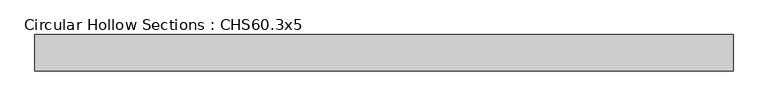
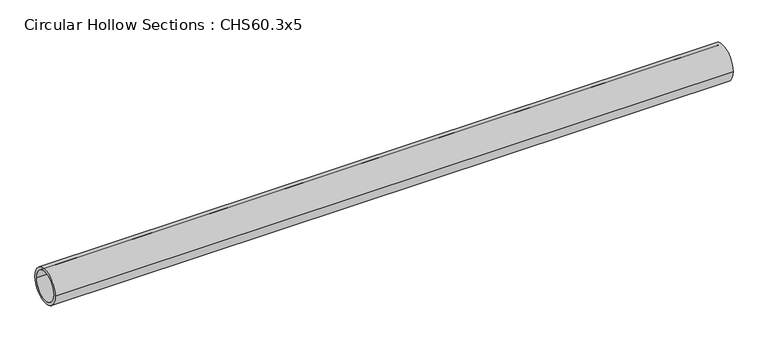
"""IFC4 building model written with IfcOpenShell, lengths in millimetres: beam geometry, Circular Hollow Sections : CHS60.3x5."""

from ifc_helpers import new_model, si_unit, point, frame, origin, origin_2d, place, context, project, spatial, circle_curve, trimmed, segment, composite_curve, outline, extrude, source, transform, mapped, element, save


def circular_hollow_sections_chs60_3x5_7809bf4e(model_context):
    return source(origin(), model_context, "Body", "SweptSolid", [
        extrude(outline(composite_curve([segment(trimmed(circle_curve(origin_2d(), 30.15), [point((-30.15, 0.0))], [point((30.15, 0.0))], False, "CARTESIAN"), True, "CONTINUOUS"), segment(trimmed(circle_curve(origin_2d(), 30.15), [point((30.15, 0.0))], [point((-30.15, 0.0))], False, "CARTESIAN"), True, "CONTINUOUS")], self_intersect=False), holes=[composite_curve([segment(trimmed(circle_curve(origin_2d(), 25.15), [point((25.15, 0.0))], [point((-25.15, 0.0))], True, "CARTESIAN"), True, "CONTINUOUS"), segment(trimmed(circle_curve(origin_2d(), 25.15), [point((-25.15, 0.0))], [point((25.15, 0.0))], True, "CARTESIAN"), True, "CONTINUOUS")], self_intersect=False)]), frame((-600.0, 0.0, 0.0), z_axis=(1.0, 0.0, 0.0), x_axis=(0.0, 1.0, 0.0)), (0.0, 0.0, 1.0), 1157.0),
    ])


if __name__ == "__main__":
    model = new_model("IFC4")
    model_context = context("Model", 3, world=origin())
    ifc_project = project(units=[si_unit("LENGTHUNIT", "METRE", prefix="MILLI")], contexts=[model_context])
    site = spatial("IfcSite", under=ifc_project)
    building = spatial("IfcBuilding", under=site)
    placement = place(None, origin())
    circular_hollow_sections_chs60_3x5_shape = circular_hollow_sections_chs60_3x5_7809bf4e(model_context)
    element("IfcBeam", 1, ObjectType="Circular Hollow Sections : CHS60.3x5", at=placement, inside=building, context=model_context, shape_type="MappedRepresentation", body=[
        mapped(circular_hollow_sections_chs60_3x5_shape, transform((0.0, 0.0, 0.0), x_axis=(1.0, 0.0, 0.0), y_axis=(0.0, 1.0, 0.0), z_axis=(0.0, 0.0, 1.0))),
    ])
    save(model, "model.ifc")

# Revit data of these elements
# Type "Circular Hollow Sections : CHS60.3x5"
#   Description = "Hollow Core Steel Roof Truss Member"
#   Type Comments = "Steel 50-355"
#   Assembly Code = "F10"
#   t = 5 mm
#   W = 0.00682
#   Start Extension Calculation [instance default] = 3000 mm
#   Start Extension [instance default] = -12.7 mm
#   Length [instance default] = 1500 mm
#   OD = 60.3 mm
#   End Extension Calculation [instance default] = 3000 mm
#   End Extension [instance default] = -12.7 mm
#   A = 0.000869 m²
#   Structural Material [instance default] = Metal - Steel 50-355
# Element 1 (IfcBeam, "Circular Hollow Sections : CHS60.3x5")
#   Materials on its faces: "Metal - Steel 50-355"
# Materials
#   "Metal - Steel 50-355": class "Metal", colour RGB 247 247 247, transparency 0
